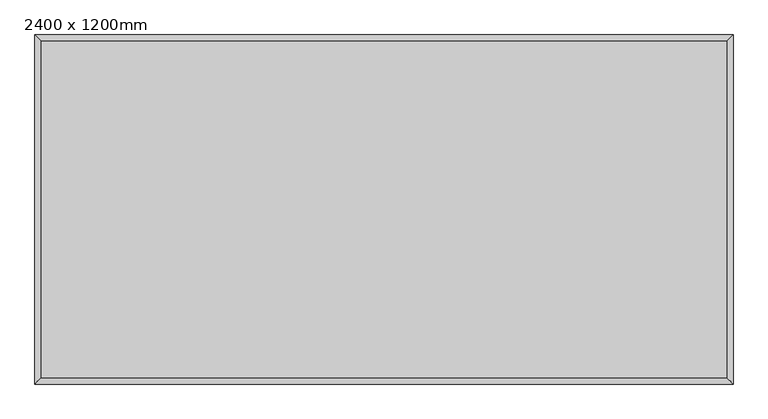
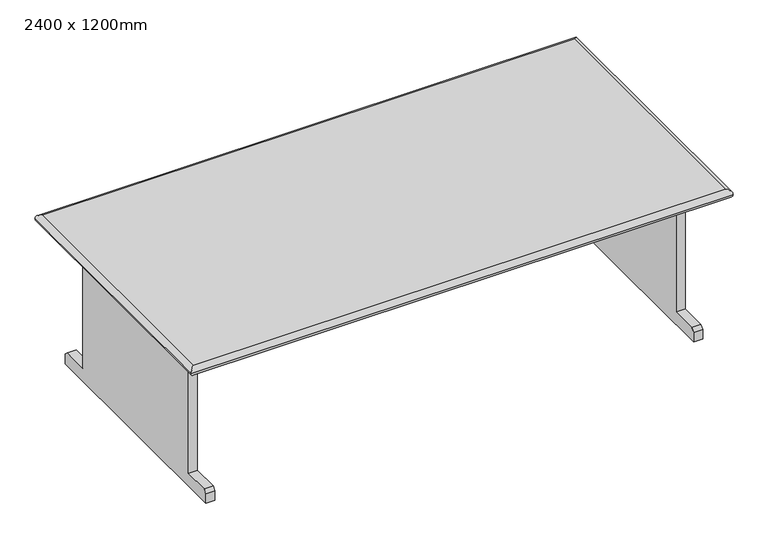
"""IFC4 building model written with IfcOpenShell, lengths in millimetres: furniture geometry, ダイニングテーブル : 2400 x 1200mm."""

from ifc_helpers import new_model, si_unit, frame, origin, place, context, project, spatial, polyline, ellipse_curve, outline, extrude, source, transform, mapped, element, save
from ifc_brep_helpers import plane_surface, cylinder_surface, advanced_brep


def furniture_2400_x_1200mm_9a885fa3(model_context):
    return source(origin(), model_context, "Body", "SolidModel", [
        advanced_brep(
        [(1200.0, 600.0, 680.0), (1180.0, 580.0, 700.0), (1180.0, -580.0, 700.0), (1200.0, -600.0, 680.0), (1180.0, -580.0, 660.0), (1180.0, 580.0, 660.0), (-1180.0, -580.0, 700.0), (-1200.0, -600.0, 680.0), (-1180.0, -580.0, 660.0), (-1180.0, 580.0, 700.0), (-1200.0, 600.0, 680.0), (-1180.0, 580.0, 660.0)],
        [
            (0, 1, ellipse_curve(frame((1180.0, 580.0, 680.0), z_axis=(0.7071067811865475, -0.7071067811865475, 0.0), x_axis=(0.7071067811865474, 0.7071067811865476, 0.0)), 28.2842712, 20.0)),
            (1, 2),
            (2, 3, ellipse_curve(frame((1180.0, -580.0, 680.0), z_axis=(0.7071067811865475, 0.7071067811865475, 0.0), x_axis=(-0.7071067811865474, 0.7071067811865476, 0.0)), 28.2842712, 20.0)),
            (3, 0),
            (3, 4, ellipse_curve(frame((1180.0, -580.0, 680.0), z_axis=(0.7071067811865475, 0.7071067811865475, 0.0), x_axis=(-0.7071067811865474, 0.7071067811865476, 0.0)), 28.2842712, 20.0)),
            (4, 5),
            (5, 0, ellipse_curve(frame((1180.0, 580.0, 680.0), z_axis=(0.7071067811865475, -0.7071067811865475, 0.0), x_axis=(0.7071067811865474, 0.7071067811865476, 0.0)), 28.2842712, 20.0)),
            (2, 6),
            (6, 7, ellipse_curve(frame((-1180.0, -580.0, 680.0), z_axis=(0.7071067811865475, -0.7071067811865475, 0.0), x_axis=(0.7071067811865476, 0.7071067811865474, 0.0)), 28.2842712, 20.0)),
            (7, 3),
            (7, 8, ellipse_curve(frame((-1180.0, -580.0, 680.0), z_axis=(0.7071067811865475, -0.7071067811865475, 0.0), x_axis=(0.7071067811865476, 0.7071067811865474, 0.0)), 28.2842712, 20.0)),
            (8, 4),
            (6, 9),
            (9, 10, ellipse_curve(frame((-1180.0, 580.0, 680.0), z_axis=(-0.7071067811865475, -0.7071067811865475, 0.0), x_axis=(0.7071067811865474, -0.7071067811865476, 0.0)), 28.2842712, 20.0)),
            (10, 7),
            (10, 11, ellipse_curve(frame((-1180.0, 580.0, 680.0), z_axis=(-0.7071067811865475, -0.7071067811865475, 0.0), x_axis=(0.7071067811865474, -0.7071067811865476, 0.0)), 28.2842712, 20.0)),
            (11, 8),
            (0, 10),
            (9, 1),
            (5, 11),
        ],
        [
            cylinder_surface(frame((1180.0, 580.0, 680.0), z_axis=(0.0, 1.0, 0.0), x_axis=(1.0, 0.0, 0.0)), 20.0),
            cylinder_surface(frame((1180.0, -580.0, 680.0), z_axis=(1.0, 0.0, 0.0), x_axis=(0.0, -1.0, 0.0)), 20.0),
            cylinder_surface(frame((-1180.0, -580.0, 680.0), z_axis=(0.0, -1.0, 0.0), x_axis=(-1.0, 0.0, 0.0)), 20.0),
            cylinder_surface(frame((-1180.0, 580.0, 680.0), z_axis=(-1.0, 0.0, 0.0), x_axis=(0.0, 1.0, 0.0)), 20.0),
            plane_surface(frame((-1180.0, 580.0, 700.0), z_axis=(0.0, 0.0, 1.0), x_axis=(-1.0, 0.0, 0.0))),
            plane_surface(frame((-1180.0, 580.0, 660.0), z_axis=(0.0, 0.0, -1.0), x_axis=(1.0, 0.0, 0.0))),
        ],
        [
            (0, [[1, 2, 3, 4]]),
            (0, [[-4, 5, 6, 7]]),
            (1, [[-3, 8, 9, 10]]),
            (1, [[-5, -10, 11, 12]]),
            (2, [[-9, 13, 14, 15]]),
            (2, [[-11, -15, 16, 17]]),
            (3, [[-1, 18, -14, 19]]),
            (3, [[-7, 20, -16, -18]]),
            (4, [[-2, -19, -13, -8]]),
            (5, [[-6, -12, -17, -20]]),
        ],
    ),
        extrude(outline(polyline([(-405.0, 660.0), (0.0, 660.0), (405.0, 660.0), (405.0, 60.0), (525.0, 60.0), (539.1421356, 45.8578644), (539.1421356, 0.0), (0.0, 0.0), (-539.1421356, 0.0), (-539.1421356, 45.8578644), (-525.0, 60.0), (-405.0, 60.0), (-405.0, 660.0)])), frame((1060.0, 0.0, 0.0), z_axis=(1.0, 0.0, 0.0), x_axis=(0.0, 1.0, 0.0)), (0.0, 0.0, 1.0), 40.0),
        extrude(outline(polyline([(-405.0, 660.0), (0.0, 660.0), (405.0, 660.0), (405.0, 60.0), (525.0, 60.0), (539.1421356, 45.8578644), (539.1421356, 0.0), (0.0, 0.0), (-539.1421356, 0.0), (-539.1421356, 45.8578644), (-525.0, 60.0), (-405.0, 60.0), (-405.0, 660.0)])), frame((-1100.0, 0.0, 0.0), z_axis=(1.0, 0.0, 0.0), x_axis=(0.0, 1.0, 0.0)), (0.0, 0.0, 1.0), 40.0),
    ])


if __name__ == "__main__":
    model = new_model("IFC4")
    model_context = context("Model", 3, world=origin())
    ifc_project = project(units=[si_unit("LENGTHUNIT", "METRE", prefix="MILLI")], contexts=[model_context])
    site = spatial("IfcSite", under=ifc_project)
    building = spatial("IfcBuilding", under=site)
    placement = place(None, origin())
    furniture_2400_x_1200mm_shape = furniture_2400_x_1200mm_9a885fa3(model_context)
    element("IfcFurniture", 1, ObjectType="ダイニングテーブル : 2400 x 1200mm", at=placement, inside=building, context=model_context, shape_type="MappedRepresentation", body=[
        mapped(furniture_2400_x_1200mm_shape, transform((0.0, 0.0, 0.0), x_axis=(1.0, 0.0, 0.0), y_axis=(0.0, 1.0, 0.0), z_axis=(0.0, 0.0, 1.0))),
    ])
    save(model, "model.ifc")

# Revit data of these elements
# Project information
#   プロジェクト発行日 = "発行日"
#   プロジェクト ステータス = "プロジェクト ステータス"
#   クライアント名 = "オーナ"
#   計画地住所 = "ここにアドレスを入力"
#   プロジェクト名 = "プロジェクト名"
#   プロジェクト番号 = "0001"
# Type "ダイニングテーブル : 2400 x 1200mm"
#   Keynote = "12490.BB1"
#   幅 = 2400 mm
#   奥行き = 1200 mm
#   本体 = 木目 - ナチュラル
#   Default Elevation = 0
# Element 1 (IfcFurniture, "ダイニングテーブル : 2400 x 1200mm")
#   Materials on its faces: "木目 - ナチュラル"
# Materials
#   "木目 - ナチュラル": class "木材", colour RGB 204 173 122, transparency 0, Cost = 0
